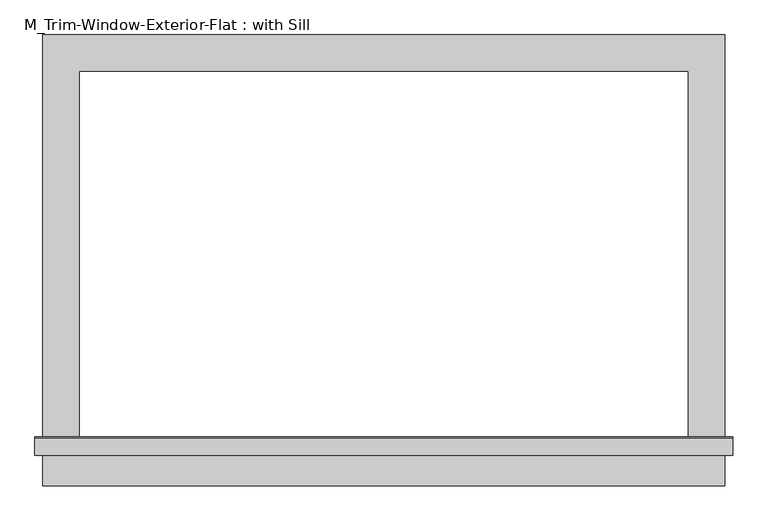
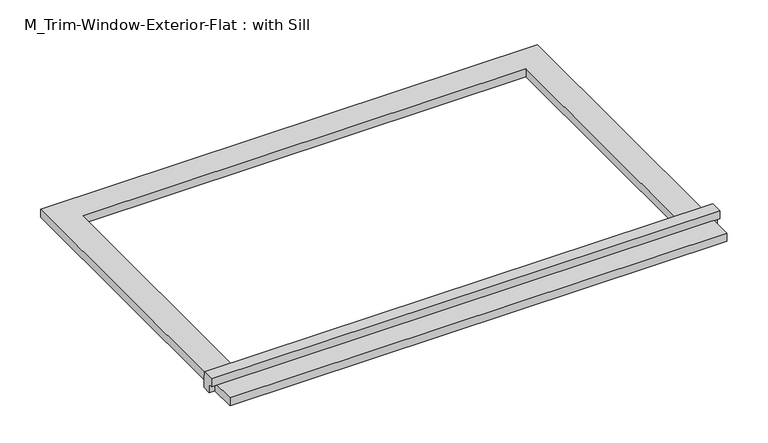
"""IFC4 building model written with IfcOpenShell, lengths in millimetres: proxy geometry, M_Trim-Window-Exterior-Flat : with Sill."""

from ifc_helpers import new_model, si_unit, frame, origin, origin_with_axes, place, context, project, spatial, polyline, outline, extrude, source, transform, mapped, element, save


def m_trim_window_exterior_flat_with_sill_c047c197(model_context):
    return source(origin(), model_context, "Body", "SweptSolid", [
        extrude(outline(polyline([(560.0, -620.4323709), (560.0, -680.4323709), (-560.0, -680.4323709), (-560.0, -620.4323709), (560.0, -620.4323709)])), origin_with_axes(), (0.0, 0.0, 1.0), 19.05),
        extrude(outline(polyline([(-630.0, 38.1), (-602.4580645, 38.1), (-600.0, 19.05), (-600.0, 0.0), (-620.4323709, 0.0), (-620.4323709, 19.05), (-630.0, 19.05), (-630.0, 38.1)])), frame((-572.7, 0.0, 0.0), z_axis=(1.0, 0.0, 0.0), x_axis=(0.0, 1.0, 0.0)), (0.0, 0.0, 1.0), 1145.4),
        extrude(outline(polyline([(-560.0, 60.0), (560.0, 60.0), (560.0, -600.0), (500.0, -600.0), (500.0, 0.0), (-500.0, 0.0), (-500.0, -600.0), (-560.0, -600.0), (-560.0, 60.0)])), origin_with_axes(), (0.0, 0.0, 1.0), 19.05),
    ])


if __name__ == "__main__":
    model = new_model("IFC4")
    model_context = context("Model", 3, world=origin())
    ifc_project = project(units=[si_unit("LENGTHUNIT", "METRE", prefix="MILLI")], contexts=[model_context])
    site = spatial("IfcSite", under=ifc_project)
    building = spatial("IfcBuilding", under=site)
    placement = place(None, origin())
    m_trim_window_exterior_flat_with_sill_shape = m_trim_window_exterior_flat_with_sill_c047c197(model_context)
    element("IfcBuildingElementProxy", 1, Name="M_Trim-Window-Exterior-Flat : with Sill", ObjectType="M_Trim-Window-Exterior-Flat : with Sill", at=placement, inside=building, context=model_context, shape_type="MappedRepresentation", body=[
        mapped(m_trim_window_exterior_flat_with_sill_shape, transform((0.0, 0.0, 0.0), x_axis=(1.0, 0.0, 0.0), y_axis=(0.0, 1.0, 0.0), z_axis=(0.0, 0.0, 1.0))),
    ])
    save(model, "model.ifc")

# Revit data of these elements
# Type "M_Trim-Window-Exterior-Flat : with Sill"
#   Trim Width = 60 mm
#   Trim Thickness_Picture Frame = 30 mm
#   Trim Thickness_with Sill = 19.05 mm
#   Sill Thickness = 30 mm
#   Opening Width [instance default] = 600 mm
#   Opening Height [instance default] = 900 mm
#   Default Elevation = 1200 mm
#   Sill = yes
#   Picture Frame = no
#   Trim Material [instance default] = none
# Element 1 (IfcBuildingElementProxy, "M_Trim-Window-Exterior-Flat : with Sill")
#   Opening Width = 1000 mm
#   Opening Height = 600 mm
#   Trim Material = Clad - White
#   Materials on its faces: "Clad - White"
# Materials
#   "Clad - White": class "Wood", colour RGB 245 245 243, transparency 0, Cost = 0
